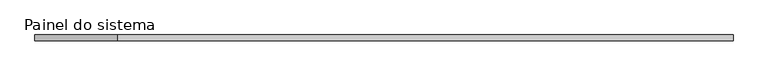
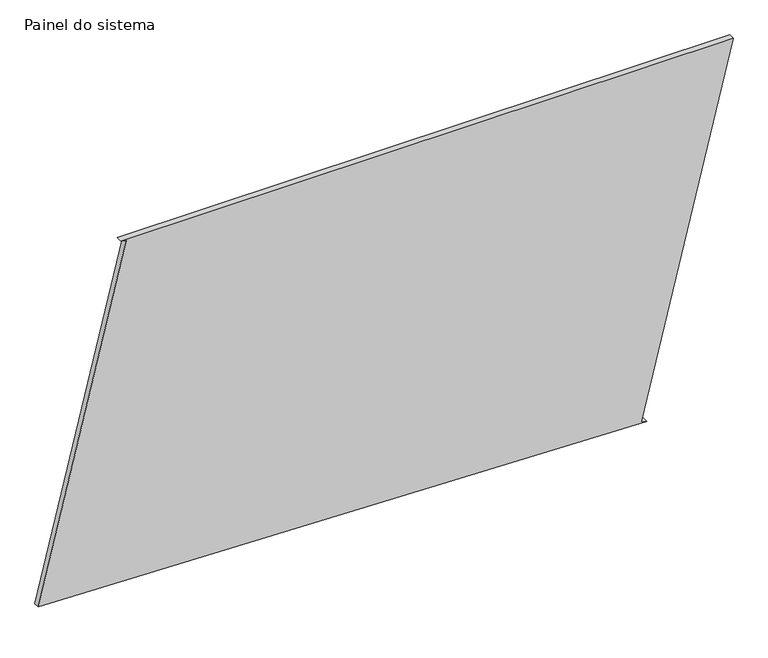
"""IFC4 building model written with IfcOpenShell, lengths in millimetres: plate geometry, Painel do sistema : Envidraçado."""

from ifc_helpers import new_model, si_unit, frame, origin, place, context, project, spatial, polyline, outline, extrude, source, transform, mapped, element, save


def painel_do_sistema_881e7d46(model_context):
    return source(origin(), model_context, "Body", "SweptSolid", [
        extrude(outline(polyline([(0.0, 1118.106908), (5.9765403, 1093.831798), (1606.9812815, 1487.9997042), (1606.9812815, -1135.7051275), (1601.0047412, -1111.4300175), (71.4792665, -1487.9997042), (0.0, 1118.106908)])), frame((0.0, 24.5, 0.0), z_axis=(0.0, 1.0, 0.0), x_axis=(0.0, 0.0, 1.0)), (0.0, 0.0, 1.0), 25.0),
    ])


if __name__ == "__main__":
    model = new_model("IFC4")
    model_context = context("Model", 3, world=origin())
    ifc_project = project(units=[si_unit("LENGTHUNIT", "METRE", prefix="MILLI")], contexts=[model_context])
    site = spatial("IfcSite", under=ifc_project)
    building = spatial("IfcBuilding", under=site)
    placement = place(None, origin())
    painel_do_sistema_shape = painel_do_sistema_881e7d46(model_context)
    element("IfcPlate", 1, ObjectType="Painel do sistema : Envidraçado", at=placement, inside=building, context=model_context, shape_type="MappedRepresentation", body=[
        mapped(painel_do_sistema_shape, transform((0.0, 0.0, 0.0), x_axis=(1.0, 0.0, 0.0), y_axis=(0.0, 1.0, 0.0), z_axis=(0.0, 0.0, 1.0))),
    ])
    save(model, "model.ifc")

# Revit data of these elements
# Type "Painel do sistema : Envidraçado"
#   Construction Type Id = "GSP4R"
#   Analytic Construction = "Vidraça única Pilkington 1/8 pol"
#   Visual Light Transmittance = 0.9
#   Solar Heat Gain Coefficient = 0.86
#   Heat Transfer Coefficient (U) = 6.7069 W/(m²·K)
# Element 1 (IfcPlate, "Painel do sistema : Envidraçado")
#   Materials on its faces: "Vidro"
# Materials
#   "Vidro": class "Vidro", colour RGB 0 128 192, transparency 0.9, Description = "Vidro de sílica", Cost = 0
